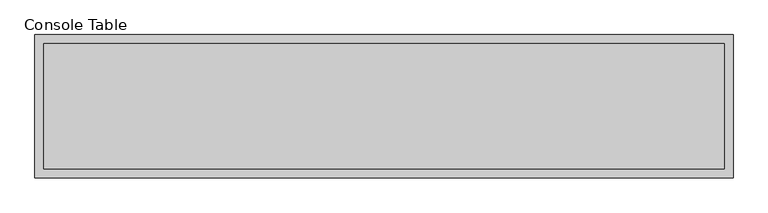
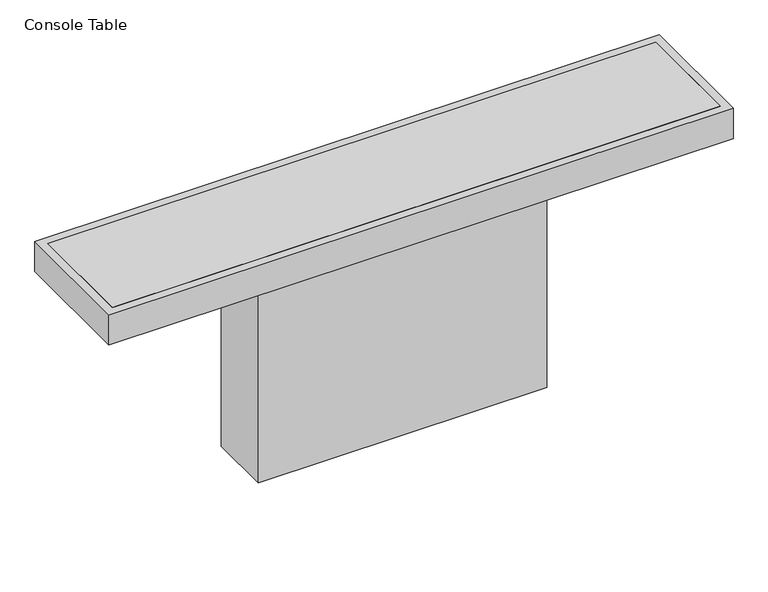
"""IFC4 building model written with IfcOpenShell, lengths in millimetres: furniture geometry, Console Table."""

import ifcopenshell
import ifcopenshell.guid

model = None  # the IFC model being written
_history = None  # IfcOwnerHistory: only IFC2X3 demands one
_inside = {}  # id of a spatial element -> (the spatial element, [elements in it])
_under = {}  # id of a project, library or spatial element -> (it, [spatial elements below it])
_declared = {}  # id of a project -> (the project, [libraries it declares])
_typed = {}  # id of a type object -> (the type object, [elements of that type])
_made_of = {}  # id of a material, layer set ... -> (it, [elements and type objects made of it])


def new_model(schema):
    """Start an empty IFC model of exactly this schema.

    Asked for "IFC4X3", IfcOpenShell would pick the latest addendum, in which some entities
    have other attributes; the version numbers below select the first issue.
    IFC2X3 requires an IfcOwnerHistory on every rooted entity: one is made here for all.
    """
    global model, _history
    if schema == "IFC4X3":
        model = ifcopenshell.file(schema_version=(4, 3, 0, 0))
    else:
        model = ifcopenshell.file(schema=schema)
    _inside.clear()
    _under.clear()
    _declared.clear()
    _typed.clear()
    _made_of.clear()
    _history = None
    if model.schema == "IFC2X3":
        org = make("IfcOrganization", Name="unknown")
        user = make(
            "IfcPersonAndOrganization",
            ThePerson=make("IfcPerson", FamilyName="unknown"),
            TheOrganization=org,
        )
        app = make(
            "IfcApplication",
            ApplicationDeveloper=org,
            Version="unknown",
            ApplicationFullName="unknown",
            ApplicationIdentifier="unknown",
        )
        _history = make(
            "IfcOwnerHistory",
            OwningUser=user,
            OwningApplication=app,
            ChangeAction="ADDED",
            CreationDate=0,
        )
    return model


def make(cls, **values):
    """One entity of the class cls with the attributes given. An attribute that is None is left unset."""
    return model.create_entity(
        cls, **{name: value for name, value in values.items() if value is not None}
    )


def rooted(cls, **values):
    """An entity with a GlobalId (a new one), such as an element, a storey or a relation."""
    return make(cls, GlobalId=ifcopenshell.guid.new(), OwnerHistory=_history, **values)


def si_unit(unit_type, name, prefix=None):
    """IfcSIUnit, for example si_unit("LENGTHUNIT", "METRE", prefix="MILLI")."""
    return make("IfcSIUnit", UnitType=unit_type, Prefix=prefix, Name=name)


def assignment(units):
    """IfcUnitAssignment: the units of a project."""
    return None if units is None else make("IfcUnitAssignment", Units=units)


def point(xyz):
    """IfcCartesianPoint."""
    return None if xyz is None else make("IfcCartesianPoint", Coordinates=xyz)


def direction(xyz):
    """IfcDirection."""
    return None if xyz is None else make("IfcDirection", DirectionRatios=xyz)


def frame(location, z_axis=None, x_axis=None):
    """IfcAxis2Placement3D, a coordinate frame: its origin and axes. An axis left out is left unset."""
    return make(
        "IfcAxis2Placement3D",
        Location=point(location),
        Axis=direction(z_axis),
        RefDirection=direction(x_axis),
    )


def origin():
    """The frame at (0, 0, 0) with its axes left unset."""
    return frame((0.0, 0.0, 0.0))


def origin_with_axes():
    """The frame at (0, 0, 0) with the z axis (0, 0, 1) and the x axis (1, 0, 0) written out."""
    return frame((0.0, 0.0, 0.0), z_axis=(0.0, 0.0, 1.0), x_axis=(1.0, 0.0, 0.0))


def place(relative_to, where):
    """IfcLocalPlacement: puts the frame where relative to a parent placement (None: the world)."""
    return make(
        "IfcLocalPlacement", PlacementRelTo=relative_to, RelativePlacement=where
    )


def context(
    kind, dimensions, precision=None, world=None, true_north=None, identifier=None
):
    """IfcGeometricRepresentationContext, for example the 3D "Model" context."""
    return make(
        "IfcGeometricRepresentationContext",
        ContextIdentifier=identifier,
        ContextType=kind,
        CoordinateSpaceDimension=dimensions,
        Precision=precision,
        WorldCoordinateSystem=world,
        TrueNorth=true_north,
    )


def project(units=None, contexts=None):
    """IfcProject with its units and contexts."""
    return rooted(
        "IfcProject",
        Name="project",
        RepresentationContexts=contexts,
        UnitsInContext=assignment(units),
    )


def spatial(cls, under=None, at=None, **own):
    """A site, building, storey or space (cls), placed at a placement, below another one or the project."""
    s = rooted(cls, ObjectPlacement=at, **own)
    if under is not None:
        _under.setdefault(under.id(), (under, []))[1].append(s)
    return s


def polyline(points):
    """IfcPolyline through the points."""
    return make("IfcPolyline", Points=[point(p) for p in points])


def outline(outer, holes=None, kind="AREA"):
    """IfcArbitraryClosedProfileDef: a profile drawn as a closed curve; with holes, ...WithVoids."""
    if holes is None:
        return make("IfcArbitraryClosedProfileDef", ProfileType=kind, OuterCurve=outer)
    return make(
        "IfcArbitraryProfileDefWithVoids",
        ProfileType=kind,
        OuterCurve=outer,
        InnerCurves=holes,
    )


def extrude(swept, where, along, depth):
    """IfcExtrudedAreaSolid: the profile swept, set in the frame where, extruded along a direction by depth."""
    return make(
        "IfcExtrudedAreaSolid",
        SweptArea=swept,
        Position=where,
        ExtrudedDirection=direction(along),
        Depth=depth,
    )


def shape(context_of_items, identifier, shape_type, items):
    """IfcShapeRepresentation: the items that make up one representation, for example the "Body"."""
    return make(
        "IfcShapeRepresentation",
        ContextOfItems=context_of_items,
        RepresentationIdentifier=identifier,
        RepresentationType=shape_type,
        Items=items,
    )


def source(mapping_origin, context_of_items, identifier, shape_type, items):
    """IfcRepresentationMap: a shape defined once, which mapped items show again and again."""
    return make(
        "IfcRepresentationMap",
        MappingOrigin=mapping_origin,
        MappedRepresentation=shape(context_of_items, identifier, shape_type, items),
    )


def transform(
    local_origin,
    x_axis=None,
    y_axis=None,
    z_axis=None,
    scale=None,
    scale2=None,
    scale3=None,
    uniform=True,
):
    """IfcCartesianTransformationOperator3D, or its non-uniform kind. x_axis, y_axis, z_axis: its Axis1, 2, 3."""
    if uniform:
        return make(
            "IfcCartesianTransformationOperator3D",
            Axis1=direction(x_axis),
            Axis2=direction(y_axis),
            LocalOrigin=point(local_origin),
            Scale=scale,
            Axis3=direction(z_axis),
        )
    return make(
        "IfcCartesianTransformationOperator3DnonUniform",
        Axis1=direction(x_axis),
        Axis2=direction(y_axis),
        LocalOrigin=point(local_origin),
        Scale=scale,
        Axis3=direction(z_axis),
        Scale2=scale2,
        Scale3=scale3,
    )


def mapped(mapping_source, mapping_target):
    """IfcMappedItem: shows the shape of a source again, moved by a transform."""
    return make(
        "IfcMappedItem", MappingSource=mapping_source, MappingTarget=mapping_target
    )


def made_of(thing, what):
    """Note that an element or type object is made of a material, layer set ...; save() writes the relation."""
    if what is not None:
        _made_of.setdefault(what.id(), (what, []))[1].append(thing)
    return thing


def element(
    cls,
    number,
    at=None,
    inside=None,
    cuts=None,
    type_object=None,
    material=None,
    context=None,
    identifier="Body",
    shape_type=None,
    held_by="IfcProductDefinitionShape",
    body=None,
    shapes=None,
    **own,
):
    """One element of the class cls, such as IfcWall. Its Tag is "e" and its number.

    at: its placement. inside: the storey or other place that contains it. cuts: it is an
    opening in that element (IfcRelVoidsElement). A single representation is given by context,
    identifier, shape_type and body (its items); several are given by shapes. held_by: the class
    of the entity that holds the representations. save() writes the other relations.
    """
    e = rooted(cls, Tag="e%d" % number, ObjectPlacement=at, **own)
    if body is not None:
        shapes = [shape(context, identifier, shape_type, body)]
    if shapes is not None:
        e.Representation = make(held_by, Representations=shapes)
    if inside is not None:
        _inside.setdefault(inside.id(), (inside, []))[1].append(e)
    if cuts is not None:
        rooted(
            "IfcRelVoidsElement", RelatingBuildingElement=cuts, RelatedOpeningElement=e
        )
    if type_object is not None:
        _typed.setdefault(type_object.id(), (type_object, []))[1].append(e)
    return made_of(e, material)


def aggregate(whole, parts):
    """IfcRelAggregates: a whole, such as a stair, and the parts it consists of."""
    return rooted("IfcRelAggregates", RelatingObject=whole, RelatedObjects=parts)


def save(model, path):
    """Write the relations noted so far, then the file.

    IfcRelAggregates (storeys below a building ...), IfcRelContainedInSpatialStructure (elements
    in a storey), IfcRelDefinesByType, IfcRelAssociatesMaterial and IfcRelDeclares: one each for
    every whole, place, type object, material and project.
    """
    for whole, parts in _under.values():
        aggregate(whole, parts)
    for where, things in _inside.values():
        rooted(
            "IfcRelContainedInSpatialStructure",
            RelatedElements=things,
            RelatingStructure=where,
        )
    for kind, things in _typed.values():
        rooted("IfcRelDefinesByType", RelatedObjects=things, RelatingType=kind)
    for what, things in _made_of.values():
        rooted("IfcRelAssociatesMaterial", RelatedObjects=things, RelatingMaterial=what)
    for by, libraries in _declared.values():
        rooted("IfcRelDeclares", RelatingContext=by, RelatedDefinitions=libraries)
    model.write(path)


def console_table_cdf4f12f(model_context):
    return source(origin(), model_context, "Body", "SweptSolid", [
        extrude(outline(polyline([(457.2, 101.6), (457.2, -101.6), (-457.2, -101.6), (-457.2, 101.6), (457.2, 101.6)])), origin_with_axes(), (0.0, 0.0, 1.0), 787.4),
        extrude(outline(polyline([(-965.2, -177.8), (-965.2, 177.8), (965.2, 177.8), (965.2, -177.8), (-965.2, -177.8)])), frame((0.0, 0.0, 787.4), z_axis=(0.0, 0.0, 1.0), x_axis=(1.0, 0.0, 0.0)), (0.0, 0.0, 1.0), 25.4),
        extrude(outline(polyline([(990.6, 203.2), (990.6, -203.2), (-990.6, -203.2), (-990.6, 203.2), (990.6, 203.2)]), holes=[polyline([(965.2, 177.8), (-965.2, 177.8), (-965.2, -177.8), (965.2, -177.8), (965.2, 177.8)])]), frame((0.0, 0.0, 711.2), z_axis=(0.0, 0.0, 1.0), x_axis=(1.0, 0.0, 0.0)), (0.0, 0.0, 1.0), 101.6),
    ])


if __name__ == "__main__":
    model = new_model("IFC4")
    model_context = context("Model", 3, world=origin())
    ifc_project = project(units=[si_unit("LENGTHUNIT", "METRE", prefix="MILLI")], contexts=[model_context])
    site = spatial("IfcSite", under=ifc_project)
    building = spatial("IfcBuilding", under=site)
    placement = place(None, origin())
    console_table_shape = console_table_cdf4f12f(model_context)
    element("IfcFurniture", 1, ObjectType="Console Table : 78\" L x 16\" W x 32\" H", at=placement, inside=building, context=model_context, shape_type="MappedRepresentation", body=[
        mapped(console_table_shape, transform((0.0, 0.0, 0.0), x_axis=(1.0, 0.0, 0.0), y_axis=(0.0, 1.0, 0.0), z_axis=(0.0, 0.0, 1.0))),
    ])
    save(model, "model.ifc")

# Revit data of these elements
# Type "Console Table : 78\" L x 16\" W x 32\" H"
#   Table Width = 406.40 mm
#   Table Length = 1981.20 mm
#   Table Height = 812.80 mm
#   Pedestal Width = 203.20 mm
#   Pedestal Length = 914.40 mm
#   Frame Thickness = 25.40 mm
#   Frame Height = 101.60 mm
#   Table Surface [instance default] = none
#   Table Frame [instance default] = none
#   Pedestal [instance default] = none
#   Assembly Code = ""
